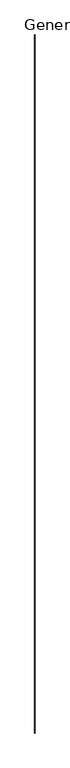
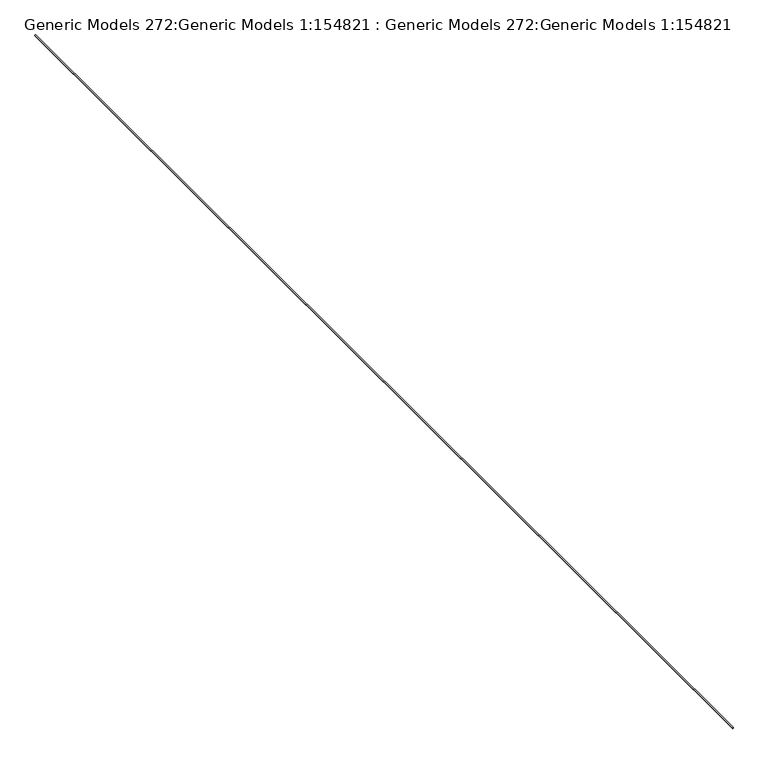
"""IFC4 building model written with IfcOpenShell, lengths in millimetres: proxy geometry, Generic Models 272:Generic Models 1:154821 : Generic Models 272:Generic Models 1:154821."""

from ifc_helpers import new_model, si_unit, point, frame, frame_2d, origin, place, context, project, spatial, polyline, circle_curve, trimmed, segment, composite_curve, outline, extrude, source, transform, mapped, element, save


def generic_models_272_generic_models_1_154821_generic_models_1da2421a(model_context):
    return source(origin(), model_context, "Body", "SweptSolid", [
        extrude(outline(composite_curve([segment(trimmed(circle_curve(frame_2d((145.7897405, 1477.5232627)), 4.3100275), [point((142.875, 1474.3482627))], [point((142.875, 1480.6982627))], False, "CARTESIAN"), True, "CONTINUOUS"), segment(polyline([(142.875, 1480.6982627), (152.4, 1480.6982627)]), True, "CONTINUOUS"), segment(trimmed(circle_curve(frame_2d((155.3147405, 1477.5232627)), 4.3100275), [point((152.4, 1480.6982627))], [point((152.4, 1474.3482627))], True, "CARTESIAN"), True, "CONTINUOUS"), segment(polyline([(152.4, 1474.3482627), (142.875, 1474.3482627)]), True, "CONTINUOUS")], self_intersect=False)), frame((0.0, -5303.1974793, 0.0), z_axis=(0.0, 1.0, 0.0), x_axis=(0.0, 0.0, 1.0)), (0.0, 0.0, 1.0), 12344.4),
    ])


if __name__ == "__main__":
    model = new_model("IFC4")
    model_context = context("Model", 3, world=origin())
    ifc_project = project(units=[si_unit("LENGTHUNIT", "METRE", prefix="MILLI")], contexts=[model_context])
    site = spatial("IfcSite", under=ifc_project)
    building = spatial("IfcBuilding", under=site)
    placement = place(None, origin())
    generic_models_272_generic_models_1_154821_generic_models_shape = generic_models_272_generic_models_1_154821_generic_models_1da2421a(model_context)
    element("IfcBuildingElementProxy", 1, Name="Generic Models 272:Generic Models 1:154821 : Generic Models 272:Generic Models 1:154821", ObjectType="Generic Models 272:Generic Models 1:154821 : Generic Models 272:Generic Models 1:154821", at=placement, inside=building, context=model_context, shape_type="MappedRepresentation", body=[
        mapped(generic_models_272_generic_models_1_154821_generic_models_shape, transform((0.0, 0.0, 0.0), x_axis=(1.0, 0.0, 0.0), y_axis=(0.0, 1.0, 0.0), z_axis=(0.0, 0.0, 1.0))),
    ])
    save(model, "model.ifc")

# Revit data of these elements
# Type "Generic Models 272:Generic Models 1:154821 : Generic Models 272:Generic Models 1:154821"
#   NameOverride = "Generic Models 272:Generic Models 1:154821"
#   ObjectTypeOverride = "Generic Models 272:Generic Models 1"
#   Reference = "Generic Models 1"
#   Category = "Generic Models"
#   Tag = "154821"
# Element 1 (IfcBuildingElementProxy, "Generic Models 272:Generic Models 1:154821 : Generic Models 272:Generic Models 1:154821")
#   Materials on its faces: "_SEALANT JOINT 27113"
# Materials
#   "_SEALANT JOINT 27113": class "Unassigned", colour RGB 190 220 196, transparency 0
